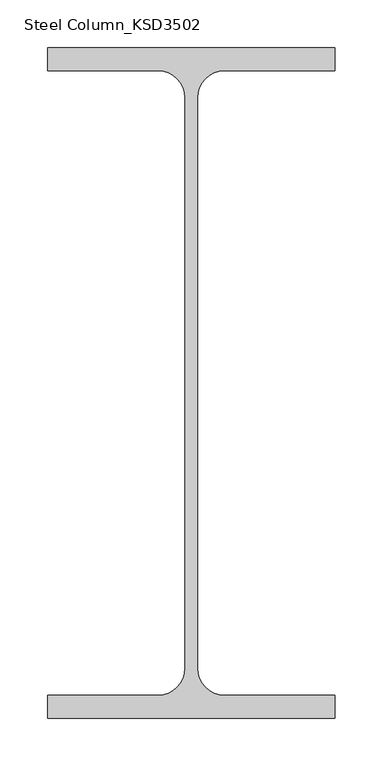
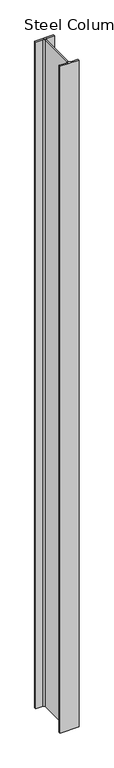
"""IFC4 building model written with IfcOpenShell, lengths in millimetres: column geometry, Steel Column_KSD3502 : H_SC_ASC_H-700×300x13x24."""

from ifc_helpers import new_model, si_unit, point, frame_2d, origin, origin_with_axes, place, context, project, spatial, polyline, circle_curve, trimmed, segment, composite_curve, outline, extrude, source, transform, mapped, element, save


def steel_column_ksd3502_ca8bed04(model_context):
    return source(origin(), model_context, "Body", "SweptSolid", [
        extrude(outline(composite_curve([segment(polyline([(150.0, 350.0), (150.0, 326.0), (34.5, 326.0)]), True, "CONTINUOUS"), segment(trimmed(circle_curve(frame_2d((34.5, 298.0)), 28.0), [point((34.5, 326.0))], [point((6.5, 298.0))], True, "CARTESIAN"), True, "CONTINUOUS"), segment(polyline([(6.5, 298.0), (6.5, -298.0)]), True, "CONTINUOUS"), segment(trimmed(circle_curve(frame_2d((34.5, -298.0)), 28.0), [point((6.5, -298.0))], [point((34.5, -326.0))], True, "CARTESIAN"), True, "CONTINUOUS"), segment(polyline([(34.5, -326.0), (150.0, -326.0), (150.0, -350.0), (-150.0, -350.0), (-150.0, -326.0), (-34.5, -326.0)]), True, "CONTINUOUS"), segment(trimmed(circle_curve(frame_2d((-34.5, -298.0)), 28.0), [point((-34.5, -326.0))], [point((-6.5, -298.0))], True, "CARTESIAN"), True, "CONTINUOUS"), segment(polyline([(-6.5, -298.0), (-6.5, 298.0)]), True, "CONTINUOUS"), segment(trimmed(circle_curve(frame_2d((-34.5, 298.0)), 28.0), [point((-6.5, 298.0))], [point((-34.5, 326.0))], True, "CARTESIAN"), True, "CONTINUOUS"), segment(polyline([(-34.5, 326.0), (-150.0, 326.0), (-150.0, 350.0), (150.0, 350.0)]), True, "CONTINUOUS")], self_intersect=False)), origin_with_axes(), (0.0, 0.0, 1.0), 11224.0),
    ])


if __name__ == "__main__":
    model = new_model("IFC4")
    model_context = context("Model", 3, world=origin())
    ifc_project = project(units=[si_unit("LENGTHUNIT", "METRE", prefix="MILLI")], contexts=[model_context])
    site = spatial("IfcSite", under=ifc_project)
    building = spatial("IfcBuilding", under=site)
    placement = place(None, origin())
    steel_column_ksd3502_shape = steel_column_ksd3502_ca8bed04(model_context)
    element("IfcColumn", 1, ObjectType="Steel Column_KSD3502 : H_SC_ASC_H-700×300x13x24", at=placement, inside=building, context=model_context, shape_type="MappedRepresentation", body=[
        mapped(steel_column_ksd3502_shape, transform((0.0, 0.0, 0.0), x_axis=(1.0, 0.0, 0.0), y_axis=(0.0, 1.0, 0.0), z_axis=(0.0, 0.0, 1.0))),
    ])
    save(model, "model.ifc")

# Revit data of these elements
# Type "Steel Column_KSD3502 : H_SC_ASC_H-700×300x13x24"
#   Width = 30.0 cm
#   Web Thickness = 1.3 cm
#   Web Fillet = 2.8 cm
#   Warping Constant = 12338400.0 cm⁶
#   Torsional Moment of Inertia = 325.986 cm⁴
#   Section Area = 235.5 cm²
#   Plastic Modulus weak axis = 1120.0 cm³
#   Plastic Modulus strong axis = 6460.0 cm³
#   Perimeter = 1.27 m²/m
#   Nominal Weight = 185.00 kgf/m
#   Moment of Inertia weak axis = 10800.00 cm⁴
#   Moment of Inertia strong axis = 201000.00 cm⁴
#   Height = 70.0 cm
#   Flange Thickness = 2.4 cm
#   Elastic Modulus weak axis = 722.0 cm³
#   Elastic Modulus strong axis = 5760.0 cm³
#   Centroid Vertical = 35.0 cm
#   Centroid Horizontal = 15.0 cm
#   Bolt Spacing = 13.97 cm
#   Structural Material [instance default] = Steel, 45-345
#   Section Name Key = ""
#   Assembly Code = ""
# Element 1 (IfcColumn, "Steel Column_KSD3502 : H_SC_ASC_H-700×300x13x24")
#   Structural Material = A03AD029-00008_Anchor Bolt (Installation only)_M36
#   Materials on its faces: "A03AD029-00008_Anchor Bolt (Installation only)_M36"
# Materials
#   "Steel, 45-345": class "Metal", colour RGB 189 187 185, transparency 0, Description = "Steel 345 MPa", Cost = 0
#   "A03AD029-00008_Anchor Bolt (Installation only)_M36": class "Unassigned", colour RGB 84 83 81, transparency 0, Cost = 0
